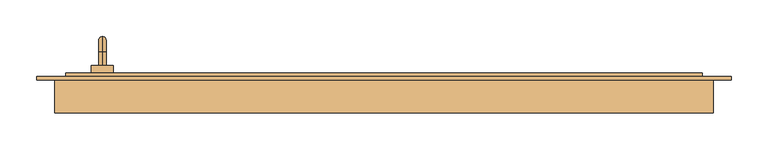
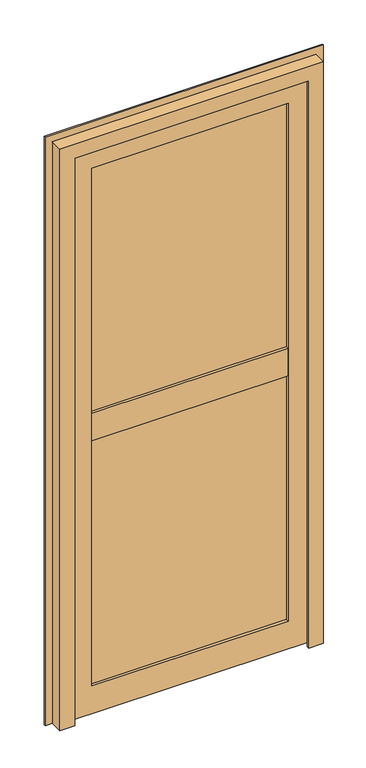
"""IFC4 building model written with IfcOpenShell, lengths in millimetres: door geometry, Puerta practicable de entrada, 1 hoja : PUERTA METALICA PABLO."""

from ifc_helpers import new_model, si_unit, point, frame, origin, place, context, project, spatial, polyline, circle_curve, ellipse_curve, trimmed, outline, extrude, faceted_brep, source, transform, mapped, element, save
from ifc_brep_helpers import plane_surface, cylinder_surface, revolved_surface, advanced_brep


def door_e94dc1a1(model_context):
    return source(origin(), model_context, "Body", "SolidModel", [
        advanced_brep(
        [(-385.0, 225.0, 905.0), (-385.0, 244.0, 905.0), (-385.0, 244.0, 895.0), (-385.0, 225.0, 895.0), (-385.0, 265.0, 884.0), (-385.0, 255.0, 884.0), (-385.0, 265.0, 805.0), (-385.0, 255.0, 805.0), (-400.0, 225.0, 930.0), (-370.0, 225.0, 930.0), (-370.0, 225.0, 870.0), (-400.0, 225.0, 870.0), (-400.0, 215.0, 930.0), (-400.0, 215.0, 870.0), (-370.0, 215.0, 870.0), (-370.0, 215.0, 930.0)],
        [
            (0, 1),
            (1, 2, circle_curve(frame((-385.0, 244.0, 900.0), z_axis=(0.0, -1.0, 0.0), x_axis=(0.0, 0.0, -1.0)), 5.0)),
            (2, 3),
            (3, 0, circle_curve(frame((-385.0, 225.0, 900.0), z_axis=(0.0, 1.0, 0.0), x_axis=(0.0, 0.0, -1.0)), 5.0)),
            (0, 3, circle_curve(frame((-385.0, 225.0, 900.0), z_axis=(0.0, 1.0, 0.0), x_axis=(0.0, 0.0, -1.0)), 5.0)),
            (2, 1, circle_curve(frame((-385.0, 244.0, 900.0), z_axis=(0.0, -1.0, 0.0), x_axis=(0.0, 0.0, -1.0)), 5.0)),
            (1, 4, circle_curve(frame((-385.0, 244.0, 884.0), z_axis=(-1.0, 0.0, 0.0), x_axis=(0.0, 0.0, 1.0)), 21.0)),
            (4, 5, circle_curve(frame((-385.0, 260.0, 884.0), z_axis=(0.0, 0.0, 1.0), x_axis=(0.0, -1.0, 0.0)), 5.0)),
            (5, 2, circle_curve(frame((-385.0, 244.0, 884.0), z_axis=(1.0, 0.0, 0.0), x_axis=(0.0, 0.0, 1.0)), 11.0)),
            (5, 4, circle_curve(frame((-385.0, 260.0, 884.0), z_axis=(0.0, 0.0, 1.0), x_axis=(0.0, -1.0, 0.0)), 5.0)),
            (6, 7, circle_curve(frame((-385.0, 260.0, 805.0), z_axis=(0.0, 0.0, -1.0), x_axis=(0.0, -1.0, 0.0)), 5.0)),
            (7, 6, circle_curve(frame((-385.0, 260.0, 805.0), z_axis=(0.0, 0.0, -1.0), x_axis=(0.0, -1.0, 0.0)), 5.0)),
            (4, 6),
            (7, 5),
            (8, 9),
            (9, 10),
            (10, 11),
            (11, 8),
            (12, 13),
            (13, 14),
            (14, 15),
            (15, 12),
            (8, 12),
            (15, 9),
            (14, 10),
            (13, 11),
        ],
        [
            cylinder_surface(frame((-385.0, 225.0, 900.0), z_axis=(0.0, -1.0, 0.0), x_axis=(0.0, 0.0, -1.0)), 5.0),
            revolved_surface(trimmed(ellipse_curve(frame((-385.0, 244.0, 900.0), z_axis=(0.0, -1.0, 0.0), x_axis=(0.0, 0.0, -1.0)), 5.0, 5.0), [point((-385.0, 244.0, 905.0))], [point((-385.0, 244.0, 895.0))], True, "CARTESIAN"), (-385.0, 244.0, 884.0), (-1.0, 0.0, 0.0)),
            revolved_surface(trimmed(ellipse_curve(frame((-385.0, 244.0, 900.0), z_axis=(0.0, -1.0, 0.0), x_axis=(0.0, 0.0, -1.0)), 5.0, 5.0), [point((-385.0, 244.0, 895.0))], [point((-385.0, 244.0, 905.0))], True, "CARTESIAN"), (-385.0, 244.0, 884.0), (-1.0, 0.0, 0.0)),
            plane_surface(frame((-385.0, 260.0, 805.0), z_axis=(0.0, 0.0, -1.0), x_axis=(-1.0, 0.0, 0.0))),
            cylinder_surface(frame((-385.0, 260.0, 884.0), z_axis=(0.0, 0.0, 1.0), x_axis=(0.0, -1.0, 0.0)), 5.0),
            plane_surface(frame((-370.0, 225.0, 930.0), z_axis=(0.0, 1.0, 0.0), x_axis=(1.0, 0.0, 0.0))),
            plane_surface(frame((-370.0, 215.0, 930.0), z_axis=(0.0, -1.0, 0.0), x_axis=(-1.0, 0.0, 0.0))),
            plane_surface(frame((-400.0, 225.0, 930.0), z_axis=(0.0, 0.0, 1.0), x_axis=(0.0, -1.0, 0.0))),
            plane_surface(frame((-370.0, 225.0, 930.0), z_axis=(1.0, 0.0, 0.0), x_axis=(0.0, -1.0, 0.0))),
            plane_surface(frame((-370.0, 225.0, 870.0), z_axis=(0.0, 0.0, -1.0), x_axis=(0.0, -1.0, 0.0))),
            plane_surface(frame((-400.0, 225.0, 870.0), z_axis=(-1.0, 0.0, 0.0), x_axis=(0.0, -1.0, 0.0))),
        ],
        [
            (0, [[1, 2, 3, 4]]),
            (0, [[-1, 5, -3, 6]]),
            (1, [[-2, 7, 8, 9]]),
            (2, [[-6, -9, 10, -7]]),
            (3, [[11, 12]]),
            (4, [[-8, 13, -12, 14]]),
            (4, [[-10, -14, -11, -13]]),
            (5, [[15, 16, 17, 18], [-4, -5]]),
            (6, [[19, 20, 21, 22]]),
            (7, [[-15, 23, -22, 24]]),
            (8, [[-16, -24, -21, 25]]),
            (9, [[-17, -25, -20, 26]]),
            (10, [[-18, -26, -19, -23]]),
        ],
    ),
        extrude(outline(polyline([(205.0, 23.0), (205.0, 8.0), (200.0, 8.0), (200.0, 13.0), (185.0, 13.0), (185.0, 8.0), (180.0, 8.0), (180.0, 23.0), (205.0, 23.0)])), frame((-435.0, 0.0, 0.0), z_axis=(1.0, 0.0, 0.0), x_axis=(0.0, 1.0, 0.0)), (0.0, 0.0, 1.0), 870.0),
        faceted_brep([(435.0, 170.0, 40.0), (435.0, 170.0, 15.0), (435.0, 180.0, 15.0), (435.0, 180.0, 40.0), (-435.0, 170.0, 40.0), (-435.0, 180.0, 40.0), (-435.0, 180.0, 15.0), (-435.0, 170.0, 15.0), (410.0, 170.0, 40.0), (410.0, 170.0, 2060.0), (-410.0, 170.0, 2060.0), (-410.0, 170.0, 40.0), (-335.0, 170.0, 1985.0), (335.0, 170.0, 1985.0), (335.0, 170.0, 115.0), (-335.0, 170.0, 115.0), (-410.0, 180.0, 40.0), (410.0, 180.0, 40.0), (-435.0, 215.0, 2085.0), (-435.0, 205.0, 2085.0), (435.0, 205.0, 2085.0), (435.0, 215.0, 2085.0), (-360.0, 180.0, 2010.0), (-360.0, 215.0, 2010.0), (360.0, 215.0, 2010.0), (360.0, 180.0, 2010.0), (-335.0, 180.0, 1985.0), (335.0, 180.0, 1985.0), (-410.0, 205.0, 2060.0), (410.0, 205.0, 2060.0), (435.0, 205.0, 15.0), (435.0, 215.0, 15.0), (360.0, 215.0, 90.0), (360.0, 180.0, 90.0), (335.0, 180.0, 115.0), (410.0, 205.0, 40.0), (-435.0, 205.0, 15.0), (-435.0, 215.0, 15.0), (-360.0, 215.0, 90.0), (-360.0, 180.0, 90.0), (-335.0, 180.0, 115.0), (-410.0, 205.0, 40.0)], [[[0, 1, 2, 3]], [[4, 5, 6, 7]], [[1, 0, 8, 9, 10, 11, 4, 7], [12, 13, 14, 15]], [[2, 1, 7, 6]], [[3, 2, 6, 5, 16, 17]], [[0, 3, 17, 8]], [[5, 4, 11, 16]], [[18, 19, 20, 21]], [[22, 23, 24, 25]], [[12, 26, 27, 13]], [[28, 10, 9, 29]], [[21, 20, 30, 31]], [[25, 24, 32, 33]], [[13, 27, 34, 14]], [[29, 9, 8, 17, 35]], [[31, 30, 36, 37]], [[33, 32, 38, 39]], [[14, 34, 40, 15]], [[41, 35, 17, 16]], [[19, 18, 37, 36]], [[18, 21, 31, 37], [24, 23, 38, 32]], [[23, 22, 39, 38]], [[22, 25, 33, 39], [27, 26, 40, 34]], [[26, 12, 15, 40]], [[10, 28, 41, 16, 11]], [[20, 19, 36, 30], [28, 29, 35, 41]]]),
        extrude(outline(polyline([(180.0, 1075.0), (215.0, 1075.0), (215.0, 1025.0), (180.0, 1025.0), (180.0, 1000.0), (170.0, 1000.0), (170.0, 1100.0), (180.0, 1100.0), (180.0, 1075.0)])), frame((-335.0, 0.0, 0.0), z_axis=(1.0, 0.0, 0.0), x_axis=(0.0, 1.0, 0.0)), (0.0, 0.0, 1.0), 670.0),
        extrude(outline(polyline([(335.0, 215.0), (335.0, 194.0), (-335.0, 194.0), (-335.0, 215.0), (335.0, 215.0)])), frame((0.0, 0.0, 1075.0), z_axis=(0.0, 0.0, 1.0), x_axis=(1.0, 0.0, 0.0)), (0.0, 0.0, 1.0), 25.0),
        extrude(outline(polyline([(335.0, 215.0), (335.0, 194.0), (-335.0, 194.0), (-335.0, 215.0), (335.0, 215.0)])), frame((0.0, 0.0, 1000.0), z_axis=(0.0, 0.0, 1.0), x_axis=(1.0, 0.0, 0.0)), (0.0, 0.0, 1.0), 25.0),
        faceted_brep([(-450.0, 160.0, 0.0), (-450.0, 205.0, 0.0), (-425.0, 205.0, 0.0), (-425.0, 170.0, 0.0), (-400.0, 170.0, 0.0), (-400.0, 160.0, 0.0), (-450.0, 160.0, 2100.0), (-450.0, 205.0, 2100.0), (450.0, 205.0, 2100.0), (450.0, 205.0, 0.0), (425.0, 205.0, 0.0), (425.0, 205.0, 2075.0), (-425.0, 205.0, 2075.0), (-425.0, 170.0, 2075.0), (425.0, 170.0, 2075.0), (425.0, 170.0, 0.0), (400.0, 170.0, 0.0), (400.0, 170.0, 2050.0), (-400.0, 170.0, 2050.0), (-400.0, 160.0, 2050.0), (400.0, 160.0, 2050.0), (400.0, 160.0, 0.0), (450.0, 160.0, 0.0), (450.0, 160.0, 2100.0)], [[[0, 1, 2, 3, 4, 5]], [[1, 0, 6, 7]], [[2, 1, 7, 8, 9, 10, 11, 12]], [[3, 2, 12, 13]], [[4, 3, 13, 14, 15, 16, 17, 18]], [[5, 4, 18, 19]], [[0, 5, 19, 20, 21, 22, 23, 6]], [[7, 6, 23, 8]], [[13, 12, 11, 14]], [[19, 18, 17, 20]], [[22, 21, 16, 15, 10, 9]], [[8, 23, 22, 9]], [[14, 11, 10, 15]], [[20, 17, 16, 21]]]),
        extrude(outline(polyline([(2010.0, -360.0), (90.0, -360.0), (90.0, 360.0), (2010.0, 360.0), (2010.0, -360.0)]), holes=[polyline([(1985.0, 335.0), (115.0, 335.0), (115.0, -335.0), (1985.0, -335.0), (1985.0, 335.0)])]), frame((0.0, 194.0, 0.0), z_axis=(0.0, 1.0, 0.0), x_axis=(0.0, 0.0, 1.0)), (0.0, 0.0, 1.0), 21.0),
        extrude(outline(polyline([(0.0, -475.0), (0.0, -440.0), (2090.0, -440.0), (2090.0, 440.0), (0.0, 440.0), (0.0, 475.0), (2125.0, 475.0), (2125.0, -475.0), (0.0, -475.0)])), frame((0.0, 205.0, 0.0), z_axis=(0.0, 1.0, 0.0), x_axis=(0.0, 0.0, 1.0)), (0.0, 0.0, 1.0), 5.0),
        extrude(outline(polyline([(350.0, 194.0), (350.0, 180.0), (-350.0, 180.0), (-350.0, 194.0), (350.0, 194.0)])), frame((0.0, 0.0, 1085.0), z_axis=(0.0, 0.0, 1.0), x_axis=(1.0, 0.0, 0.0)), (0.0, 0.0, 1.0), 915.0),
        extrude(outline(polyline([(350.0, 194.0), (350.0, 180.0), (-350.0, 180.0), (-350.0, 194.0), (350.0, 194.0)])), frame((0.0, 0.0, 100.0), z_axis=(0.0, 0.0, 1.0), x_axis=(1.0, 0.0, 0.0)), (0.0, 0.0, 1.0), 915.0),
    ])


if __name__ == "__main__":
    model = new_model("IFC4")
    model_context = context("Model", 3, world=origin())
    ifc_project = project(units=[si_unit("LENGTHUNIT", "METRE", prefix="MILLI")], contexts=[model_context])
    site = spatial("IfcSite", under=ifc_project)
    building = spatial("IfcBuilding", under=site)
    placement = place(None, origin())
    door_shape = door_e94dc1a1(model_context)
    element("IfcDoor", 1, ObjectType="Puerta practicable de entrada, 1 hoja : PUERTA METALICA PABLO", at=placement, inside=building, context=model_context, shape_type="MappedRepresentation", body=[
        mapped(door_shape, transform((0.0, 0.0, 0.0), x_axis=(1.0, 0.0, 0.0), y_axis=(0.0, 1.0, 0.0), z_axis=(0.0, 0.0, 1.0))),
    ])
    save(model, "model.ifc")

# Revit data of these elements
# Type "Puerta practicable de entrada, 1 hoja : PUERTA METALICA PABLO"
#   Description = "Puerta metálica 1 hoja abatible"
#   Type Mark = "P1"
#   Construction Type Id = "MDOOR"
#   Analytic Construction = "Metal"
#   w = 0.015 m
#   Anchura de cubrejuntas = 0.035 m
#   Grosor de cubrejuntas = 0.005 m
#   Rough Width = 0.90 m
#   Rough Height = 2.10 m
#   Anchura de panel = 0.87 m
#   Anchura de marco de panel = 0.10 m
#   Heat Transfer Coefficient (U) = 3.7021 W/(m²·K)
#   Anchura de marco = 0.05 m
#   Height = 2.10 m
#   Width = 0.90 m
#   Grosor de marco = 0.045 m
#   Define Thermal Properties by = 1
#   Function = 1
#   Material de tirador = none
#   Material de cristalera = none
#   Material de estructura = none
#   Visual Light Transmittance = 0
#   Solar Heat Gain Coefficient = 0
#   Wall Closure = (empty or 0)
# Element 1 (IfcDoor, "Puerta practicable de entrada, 1 hoja : PUERTA METALICA PABLO")
#   Materials on its faces: "Madera - Castaño", "Vidrio"
# Materials
#   "Madera - Castaño": class "Madera", colour RGB 190 129 78, transparency 0, Cost = 0
#   "Vidrio": class "Vidrio", colour RGB 0 128 192, transparency 0.75, Description = "Vidrio de cal sodada", Cost = 0
